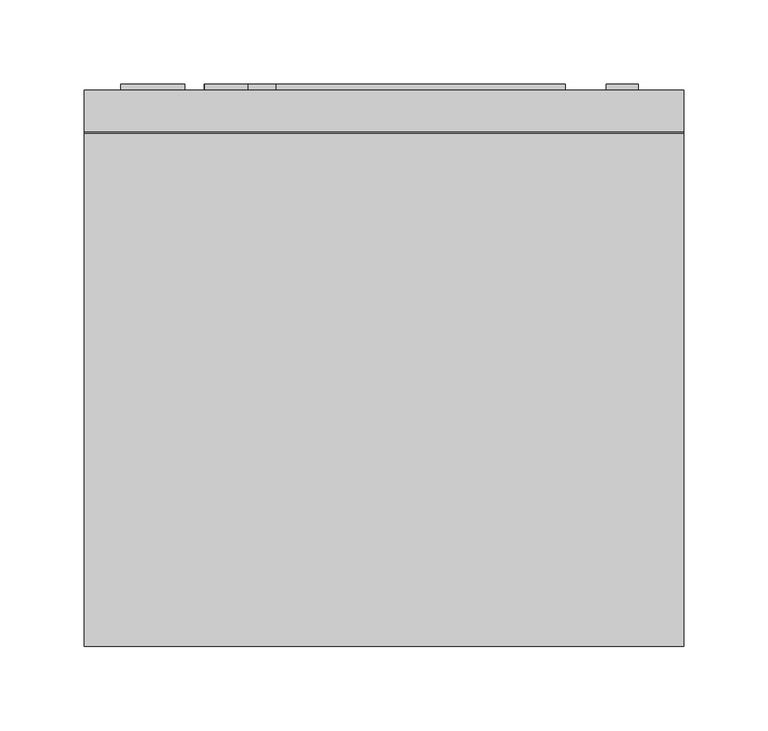
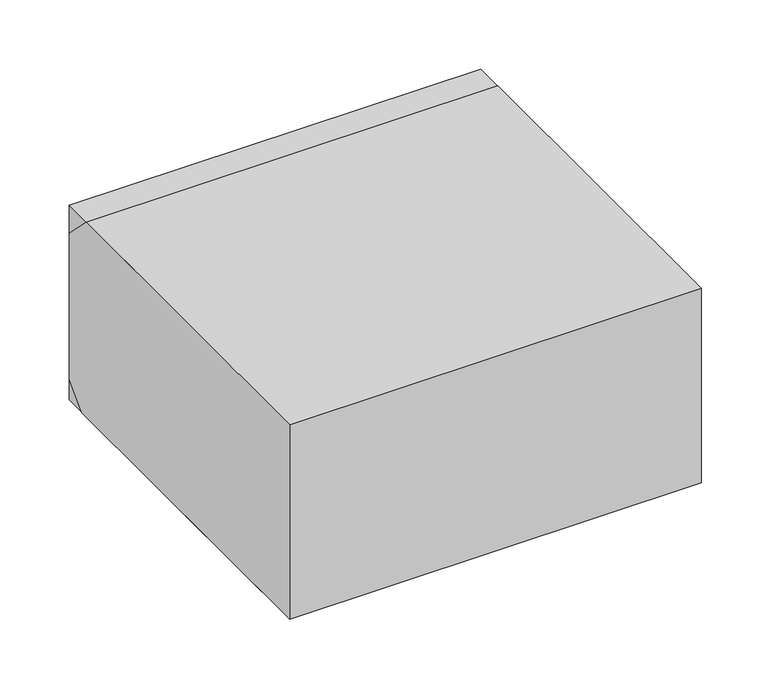
"""IFC4 building model written with IfcOpenShell, lengths in millimetres: proxy geometry, M8555 - Insufflator, Automatic Controls : M8555 - Insufflator, Automatic Controls."""

import ifcopenshell
import ifcopenshell.guid

model = None  # the IFC model being written
_history = None  # IfcOwnerHistory: only IFC2X3 demands one
_inside = {}  # id of a spatial element -> (the spatial element, [elements in it])
_under = {}  # id of a project, library or spatial element -> (it, [spatial elements below it])
_declared = {}  # id of a project -> (the project, [libraries it declares])
_typed = {}  # id of a type object -> (the type object, [elements of that type])
_made_of = {}  # id of a material, layer set ... -> (it, [elements and type objects made of it])


def new_model(schema):
    """Start an empty IFC model of exactly this schema.

    Asked for "IFC4X3", IfcOpenShell would pick the latest addendum, in which some entities
    have other attributes; the version numbers below select the first issue.
    IFC2X3 requires an IfcOwnerHistory on every rooted entity: one is made here for all.
    """
    global model, _history
    if schema == "IFC4X3":
        model = ifcopenshell.file(schema_version=(4, 3, 0, 0))
    else:
        model = ifcopenshell.file(schema=schema)
    _inside.clear()
    _under.clear()
    _declared.clear()
    _typed.clear()
    _made_of.clear()
    _history = None
    if model.schema == "IFC2X3":
        org = make("IfcOrganization", Name="unknown")
        user = make(
            "IfcPersonAndOrganization",
            ThePerson=make("IfcPerson", FamilyName="unknown"),
            TheOrganization=org,
        )
        app = make(
            "IfcApplication",
            ApplicationDeveloper=org,
            Version="unknown",
            ApplicationFullName="unknown",
            ApplicationIdentifier="unknown",
        )
        _history = make(
            "IfcOwnerHistory",
            OwningUser=user,
            OwningApplication=app,
            ChangeAction="ADDED",
            CreationDate=0,
        )
    return model


def make(cls, **values):
    """One entity of the class cls with the attributes given. An attribute that is None is left unset."""
    return model.create_entity(
        cls, **{name: value for name, value in values.items() if value is not None}
    )


def rooted(cls, **values):
    """An entity with a GlobalId (a new one), such as an element, a storey or a relation."""
    return make(cls, GlobalId=ifcopenshell.guid.new(), OwnerHistory=_history, **values)


def si_unit(unit_type, name, prefix=None):
    """IfcSIUnit, for example si_unit("LENGTHUNIT", "METRE", prefix="MILLI")."""
    return make("IfcSIUnit", UnitType=unit_type, Prefix=prefix, Name=name)


def assignment(units):
    """IfcUnitAssignment: the units of a project."""
    return None if units is None else make("IfcUnitAssignment", Units=units)


def point(xyz):
    """IfcCartesianPoint."""
    return None if xyz is None else make("IfcCartesianPoint", Coordinates=xyz)


def direction(xyz):
    """IfcDirection."""
    return None if xyz is None else make("IfcDirection", DirectionRatios=xyz)


def frame(location, z_axis=None, x_axis=None):
    """IfcAxis2Placement3D, a coordinate frame: its origin and axes. An axis left out is left unset."""
    return make(
        "IfcAxis2Placement3D",
        Location=point(location),
        Axis=direction(z_axis),
        RefDirection=direction(x_axis),
    )


def origin():
    """The frame at (0, 0, 0) with its axes left unset."""
    return frame((0.0, 0.0, 0.0))


def origin_with_axes():
    """The frame at (0, 0, 0) with the z axis (0, 0, 1) and the x axis (1, 0, 0) written out."""
    return frame((0.0, 0.0, 0.0), z_axis=(0.0, 0.0, 1.0), x_axis=(1.0, 0.0, 0.0))


def place(relative_to, where):
    """IfcLocalPlacement: puts the frame where relative to a parent placement (None: the world)."""
    return make(
        "IfcLocalPlacement", PlacementRelTo=relative_to, RelativePlacement=where
    )


def context(
    kind, dimensions, precision=None, world=None, true_north=None, identifier=None
):
    """IfcGeometricRepresentationContext, for example the 3D "Model" context."""
    return make(
        "IfcGeometricRepresentationContext",
        ContextIdentifier=identifier,
        ContextType=kind,
        CoordinateSpaceDimension=dimensions,
        Precision=precision,
        WorldCoordinateSystem=world,
        TrueNorth=true_north,
    )


def project(units=None, contexts=None):
    """IfcProject with its units and contexts."""
    return rooted(
        "IfcProject",
        Name="project",
        RepresentationContexts=contexts,
        UnitsInContext=assignment(units),
    )


def spatial(cls, under=None, at=None, **own):
    """A site, building, storey or space (cls), placed at a placement, below another one or the project."""
    s = rooted(cls, ObjectPlacement=at, **own)
    if under is not None:
        _under.setdefault(under.id(), (under, []))[1].append(s)
    return s


def polyline(points):
    """IfcPolyline through the points."""
    return make("IfcPolyline", Points=[point(p) for p in points])


def outline(outer, holes=None, kind="AREA"):
    """IfcArbitraryClosedProfileDef: a profile drawn as a closed curve; with holes, ...WithVoids."""
    if holes is None:
        return make("IfcArbitraryClosedProfileDef", ProfileType=kind, OuterCurve=outer)
    return make(
        "IfcArbitraryProfileDefWithVoids",
        ProfileType=kind,
        OuterCurve=outer,
        InnerCurves=holes,
    )


def extrude(swept, where, along, depth):
    """IfcExtrudedAreaSolid: the profile swept, set in the frame where, extruded along a direction by depth."""
    return make(
        "IfcExtrudedAreaSolid",
        SweptArea=swept,
        Position=where,
        ExtrudedDirection=direction(along),
        Depth=depth,
    )


def shape(context_of_items, identifier, shape_type, items):
    """IfcShapeRepresentation: the items that make up one representation, for example the "Body"."""
    return make(
        "IfcShapeRepresentation",
        ContextOfItems=context_of_items,
        RepresentationIdentifier=identifier,
        RepresentationType=shape_type,
        Items=items,
    )


def source(mapping_origin, context_of_items, identifier, shape_type, items):
    """IfcRepresentationMap: a shape defined once, which mapped items show again and again."""
    return make(
        "IfcRepresentationMap",
        MappingOrigin=mapping_origin,
        MappedRepresentation=shape(context_of_items, identifier, shape_type, items),
    )


def transform(
    local_origin,
    x_axis=None,
    y_axis=None,
    z_axis=None,
    scale=None,
    scale2=None,
    scale3=None,
    uniform=True,
):
    """IfcCartesianTransformationOperator3D, or its non-uniform kind. x_axis, y_axis, z_axis: its Axis1, 2, 3."""
    if uniform:
        return make(
            "IfcCartesianTransformationOperator3D",
            Axis1=direction(x_axis),
            Axis2=direction(y_axis),
            LocalOrigin=point(local_origin),
            Scale=scale,
            Axis3=direction(z_axis),
        )
    return make(
        "IfcCartesianTransformationOperator3DnonUniform",
        Axis1=direction(x_axis),
        Axis2=direction(y_axis),
        LocalOrigin=point(local_origin),
        Scale=scale,
        Axis3=direction(z_axis),
        Scale2=scale2,
        Scale3=scale3,
    )


def mapped(mapping_source, mapping_target):
    """IfcMappedItem: shows the shape of a source again, moved by a transform."""
    return make(
        "IfcMappedItem", MappingSource=mapping_source, MappingTarget=mapping_target
    )


def made_of(thing, what):
    """Note that an element or type object is made of a material, layer set ...; save() writes the relation."""
    if what is not None:
        _made_of.setdefault(what.id(), (what, []))[1].append(thing)
    return thing


def element(
    cls,
    number,
    at=None,
    inside=None,
    cuts=None,
    type_object=None,
    material=None,
    context=None,
    identifier="Body",
    shape_type=None,
    held_by="IfcProductDefinitionShape",
    body=None,
    shapes=None,
    **own,
):
    """One element of the class cls, such as IfcWall. Its Tag is "e" and its number.

    at: its placement. inside: the storey or other place that contains it. cuts: it is an
    opening in that element (IfcRelVoidsElement). A single representation is given by context,
    identifier, shape_type and body (its items); several are given by shapes. held_by: the class
    of the entity that holds the representations. save() writes the other relations.
    """
    e = rooted(cls, Tag="e%d" % number, ObjectPlacement=at, **own)
    if body is not None:
        shapes = [shape(context, identifier, shape_type, body)]
    if shapes is not None:
        e.Representation = make(held_by, Representations=shapes)
    if inside is not None:
        _inside.setdefault(inside.id(), (inside, []))[1].append(e)
    if cuts is not None:
        rooted(
            "IfcRelVoidsElement", RelatingBuildingElement=cuts, RelatedOpeningElement=e
        )
    if type_object is not None:
        _typed.setdefault(type_object.id(), (type_object, []))[1].append(e)
    return made_of(e, material)


def aggregate(whole, parts):
    """IfcRelAggregates: a whole, such as a stair, and the parts it consists of."""
    return rooted("IfcRelAggregates", RelatingObject=whole, RelatedObjects=parts)


def save(model, path):
    """Write the relations noted so far, then the file.

    IfcRelAggregates (storeys below a building ...), IfcRelContainedInSpatialStructure (elements
    in a storey), IfcRelDefinesByType, IfcRelAssociatesMaterial and IfcRelDeclares: one each for
    every whole, place, type object, material and project.
    """
    for whole, parts in _under.values():
        aggregate(whole, parts)
    for where, things in _inside.values():
        rooted(
            "IfcRelContainedInSpatialStructure",
            RelatedElements=things,
            RelatingStructure=where,
        )
    for kind, things in _typed.values():
        rooted("IfcRelDefinesByType", RelatedObjects=things, RelatingType=kind)
    for what, things in _made_of.values():
        rooted("IfcRelAssociatesMaterial", RelatedObjects=things, RelatingMaterial=what)
    for by, libraries in _declared.values():
        rooted("IfcRelDeclares", RelatingContext=by, RelatedDefinitions=libraries)
    model.write(path)


def specialty_equipment_ec502b29(model_context):
    return source(origin(), model_context, "Body", "SweptSolid", [
        extrude(outline(polyline([(-118.1220681, 165.1), (-156.2220681, 165.1), (-156.2220681, 168.6216965), (-118.1220681, 168.6216965), (-118.1220681, 165.1)])), frame((0.0, 0.0, 32.8532625), z_axis=(0.0, 0.0, 1.0), x_axis=(1.0, 0.0, 0.0)), (0.0, 0.0, 1.0), 107.95),
        extrude(outline(polyline([(0.0, 165.1), (-106.5512543, 165.1), (-106.5512543, 168.6216965), (0.0, 168.6216965), (0.0, 165.1)])), frame((0.0, 0.0, 32.6606569), z_axis=(0.0, 0.0, 1.0), x_axis=(1.0, 0.0, 0.0)), (0.0, 0.0, 1.0), 34.7124413),
        extrude(outline(polyline([(-80.9681755, 165.1), (-106.3681755, 165.1), (-106.3681755, 168.6216965), (-80.9681755, 168.6216965), (-80.9681755, 165.1)])), frame((0.0, 0.0, 83.4898148), z_axis=(0.0, 0.0, 1.0), x_axis=(1.0, 0.0, 0.0)), (0.0, 0.0, 1.0), 19.05),
        extrude(outline(polyline([(-80.9681755, 165.1), (-106.3681755, 165.1), (-106.3681755, 168.6216965), (-80.9681755, 168.6216965), (-80.9681755, 165.1)])), frame((0.0, 0.0, 121.5898148), z_axis=(0.0, 0.0, 1.0), x_axis=(1.0, 0.0, 0.0)), (0.0, 0.0, 1.0), 19.05),
        extrude(outline(polyline([(107.4091764, 165.1), (-64.0408236, 165.1), (-64.0408236, 168.6216965), (107.4091764, 168.6216965), (107.4091764, 165.1)])), frame((0.0, 0.0, 82.4604304), z_axis=(0.0, 0.0, 1.0), x_axis=(1.0, 0.0, 0.0)), (0.0, 0.0, 1.0), 19.05),
        extrude(outline(polyline([(107.4091764, 165.1), (-64.0408236, 165.1), (-64.0408236, 168.6216965), (107.4091764, 168.6216965), (107.4091764, 165.1)])), frame((0.0, 0.0, 120.5604304), z_axis=(0.0, 0.0, 1.0), x_axis=(1.0, 0.0, 0.0)), (0.0, 0.0, 1.0), 19.05),
        extrude(outline(polyline([(150.8026816, 165.1), (131.7526816, 165.1), (131.7526816, 168.6216965), (150.8026816, 168.6216965), (150.8026816, 165.1)])), frame((0.0, 0.0, 76.8229594), z_axis=(0.0, 0.0, 1.0), x_axis=(1.0, 0.0, 0.0)), (0.0, 0.0, 1.0), 63.5),
        extrude(outline(polyline([(150.8026816, 165.1), (131.7526816, 165.1), (131.7526816, 168.6216965), (150.8026816, 168.6216965), (150.8026816, 165.1)])), frame((0.0, 0.0, 29.9056647), z_axis=(0.0, 0.0, 1.0), x_axis=(1.0, 0.0, 0.0)), (0.0, 0.0, 1.0), 31.75),
        extrude(outline(polyline([(-165.1, 0.0), (-165.1, 177.8), (139.7, 177.8), (165.1, 152.4), (165.1, 19.05), (146.05, 0.0), (-165.1, 0.0)])), frame((-177.8, 0.0, 0.0), z_axis=(1.0, 0.0, 0.0), x_axis=(0.0, 1.0, 0.0)), (0.0, 0.0, 1.0), 355.6),
        extrude(outline(polyline([(-177.8, 165.1), (177.8, 165.1), (177.8, -165.1), (-177.8, -165.1), (-177.8, 0.0), (-177.8, 165.1)])), origin_with_axes(), (0.0, 0.0, 1.0), 177.8),
    ])


if __name__ == "__main__":
    model = new_model("IFC4")
    model_context = context("Model", 3, world=origin())
    ifc_project = project(units=[si_unit("LENGTHUNIT", "METRE", prefix="MILLI")], contexts=[model_context])
    site = spatial("IfcSite", under=ifc_project)
    building = spatial("IfcBuilding", under=site)
    placement = place(None, origin())
    specialty_equipment_shape = specialty_equipment_ec502b29(model_context)
    element("IfcBuildingElementProxy", 1, Name="M8555 - Insufflator, Automatic Controls : M8555 - Insufflator, Automatic Controls", ObjectType="M8555 - Insufflator, Automatic Controls : M8555 - Insufflator, Automatic Controls", at=placement, inside=building, context=model_context, shape_type="MappedRepresentation", body=[
        mapped(specialty_equipment_shape, transform((0.0, 0.0, 0.0), x_axis=(1.0, 0.0, 0.0), y_axis=(0.0, 1.0, 0.0), z_axis=(0.0, 0.0, 1.0))),
    ])
    save(model, "model.ifc")

# Revit data of these elements
# Type "M8555 - Insufflator, Automatic Controls : M8555 - Insufflator, Automatic Controls"
#   Watts2 = "0"
#   Watts1 = "120"
#   Unit_Issue = "EA"
#   UTIL_6_Misc = "-"
#   UTIL_5_NonMedGas = "-"
#   UTIL_4_MiscGas = "E"
#   UTIL_3_MedGas = "-"
#   UTIL_2_Elec = "A"
#   UTIL_1_WaterDrain = "-"
#   Nomenclature = "Insufflator, Automatic Controls"
#   NSN = "6515"
#   Location [instance default] = ""
#   JSN = "M8555"
#   Fund_Source_VA = "-"
#   Fund_Source_Navy = "-"
#   Fund_Source_Army = "-"
#   Fund_Source_AF = "-"
#   ELEC_Volts2 = "0"
#   ELEC_Volts1 = "120"
#   ELEC_Phase2 = "0"
#   ELEC_Phase1 = "1"
#   ELEC_HertzSwitch = "0"
#   ELEC_HertzDependent = "-1"
#   ELEC_Hertz = "600"
#   ELEC_Amps2 = "0"
#   ELEC_Amps1 = "1"
#   DetailDescription = "Automatic controlled insufflator is used to infuse CO2 during endoscopic and laser surgery. Unit provides controlled pressure of CO2 within the cavity of interest and eliminates air from the site. This item is also a component of the JSN M8605-M8607 and M8610-M8611 endoscopy carts."
#   CAT_VA = "C"
#   CAT_Navy = "C"
#   CAT_IHS = "-"
#   CAT_Army = "C"
#   CAT_AF = "C"
#   BTUperhour = "0"
#   Weight_IP = 22
#   DIM_Width_IP = 1' - 2"
#   DIM_Height_IP = 0' - 7"
#   DIM_Depth_IP = 1' - 1"
# Element 1 (IfcBuildingElementProxy, "M8555 - Insufflator, Automatic Controls : M8555 - Insufflator, Automatic Controls")
#   Materials on its faces: "EquipSpace"
# Materials
#   "EquipSpace": class "Unassigned", colour RGB 221 217 195, transparency 0.5
